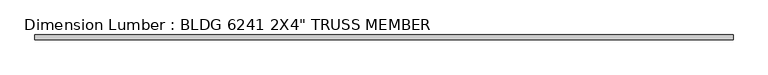
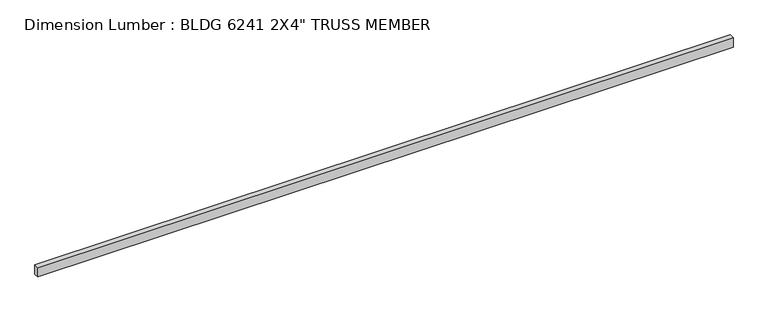
"""IFC4 building model written with IfcOpenShell, lengths in millimetres: beam geometry."""

from ifc_helpers import new_model, si_unit, frame, origin, place, context, project, spatial, polyline, outline, extrude, source, transform, mapped, element, save


def beam_44bcd8c2(model_context):
    return source(origin(), model_context, "Body", "SweptSolid", [
        extrude(outline(polyline([(3555.9999994, 25.4), (3555.9999994, -25.4), (-3555.9999994, -25.4), (-3555.9999994, 25.4), (3555.9999994, 25.4)])), frame((0.0, 0.0, -50.8), z_axis=(0.0, 0.0, 1.0), x_axis=(1.0, 0.0, 0.0)), (0.0, 0.0, 1.0), 101.6),
    ])


if __name__ == "__main__":
    model = new_model("IFC4")
    model_context = context("Model", 3, world=origin())
    ifc_project = project(units=[si_unit("LENGTHUNIT", "METRE", prefix="MILLI")], contexts=[model_context])
    site = spatial("IfcSite", under=ifc_project)
    building = spatial("IfcBuilding", under=site)
    placement = place(None, origin())
    beam_shape = beam_44bcd8c2(model_context)
    element("IfcBeam", 1, ObjectType="Dimension Lumber : BLDG 6241 2X4\" TRUSS MEMBER", at=placement, inside=building, context=model_context, shape_type="MappedRepresentation", body=[
        mapped(beam_shape, transform((0.0, 0.0, 0.0), x_axis=(1.0, 0.0, 0.0), y_axis=(0.0, 1.0, 0.0), z_axis=(0.0, 0.0, 1.0))),
    ])
    save(model, "model.ifc")

# Revit data of these elements
# Type "Dimension Lumber : BLDG 6241 2X4\" TRUSS MEMBER"
#   Assembly Code = "B10"
#   A = 0.273472 SF
#   Length [instance default] = 5' - 0"
#   b = 0' - 2"
#   d = 0' - 4"
#   Structural Material [instance default] = Softwood, Lumber
# Element 1 (IfcBeam, "Dimension Lumber : BLDG 6241 2X4\" TRUSS MEMBER")
#   Materials on its faces: "Softwood, Lumber"
# Materials
#   "Softwood, Lumber": class "Wood", colour RGB 223 192 134, transparency 0, Description = "Pinus Echinata", Cost = 0
